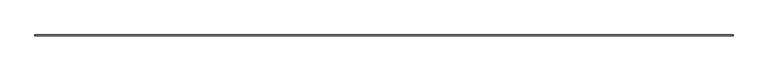
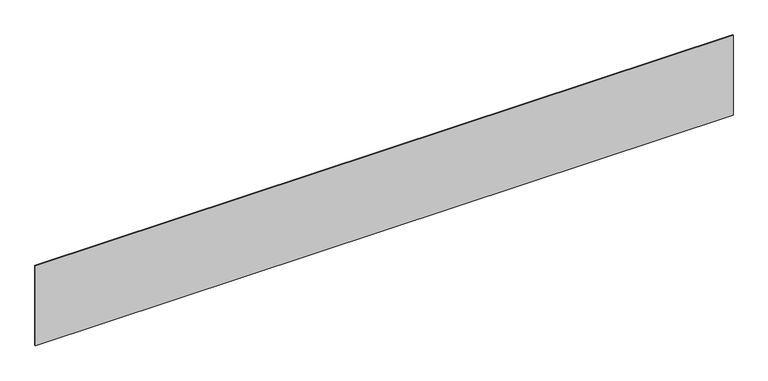
"""IFC4 building model written with IfcOpenShell, lengths in millimetres: proxy geometry, Inner panel:Inner panel:1:Inner panel:1 : Inner panel:Inner panel:300324:300043:Inner panel:1:Inner panel:1 : Inner panel:Inner panel:300324:300043 : Inner panel:Inner panel:1:Inner panel:1 : Inner panel:Inner panel:300324:300043:12 : Inner panel:Inner panel:1:Inner panel:1 : Inner panel:Inner panel:300324:300043:Inner panel:1:Inner panel:1 : Inner panel:Inner panel:300324:300043 : Inner panel:Inner panel:1:Inner panel:1 : Inner panel:Inner panel:300324:300043:300031."""

from ifc_helpers import new_model, si_unit, frame, origin, place, context, project, spatial, polyline, outline, extrude, source, transform, mapped, element, save


def generic_models_44e0b5d8(model_context):
    return source(origin(), model_context, "Body", "SweptSolid", [
        extrude(outline(polyline([(560352.9617239, -579000.6913841), (570446.2867239, -579000.6913841), (570446.2867239, -579013.3913841), (560352.9617239, -579013.3913841), (560352.9617239, -579000.6913841)])), frame((0.0, 0.0, 3721.1), z_axis=(0.0, 0.0, 1.0), x_axis=(1.0, 0.0, 0.0)), (0.0, 0.0, 1.0), 1219.2),
    ])


if __name__ == "__main__":
    model = new_model("IFC4")
    model_context = context("Model", 3, world=origin())
    ifc_project = project(units=[si_unit("LENGTHUNIT", "METRE", prefix="MILLI")], contexts=[model_context])
    site = spatial("IfcSite", under=ifc_project)
    building = spatial("IfcBuilding", under=site)
    placement = place(None, origin())
    generic_models_shape = generic_models_44e0b5d8(model_context)
    element("IfcBuildingElementProxy", 1, Name="Inner panel:Inner panel:1:Inner panel:1 : Inner panel:Inner panel:300324:300043:Inner panel:1:Inner panel:1 : Inner panel:Inner panel:300324:300043 : Inner panel:Inner panel:1:Inner panel:1 : Inner panel:Inner panel:300324:300043:12 : Inner panel:Inner panel:1:Inner panel:1 : Inner panel:Inner panel:300324:300043:Inner panel:1:Inner panel:1 : Inner panel:Inner panel:300324:300043 : Inner panel:Inner panel:1:Inner panel:1 : Inner panel:Inner panel:300324:300043:300031", ObjectType="Inner panel:Inner panel:1:Inner panel:1 : Inner panel:Inner panel:300324:300043:Inner panel:1:Inner panel:1 : Inner panel:Inner panel:300324:300043 : Inner panel:Inner panel:1:Inner panel:1 : Inner panel:Inner panel:300324:300043:12 : Inner panel:Inner panel:1:Inner panel:1 : Inner panel:Inner panel:300324:300043:Inner panel:1:Inner panel:1 : Inner panel:Inner panel:300324:300043 : Inner panel:Inner panel:1:Inner panel:1 : Inner panel:Inner panel:300324:300043:300031", at=placement, inside=building, context=model_context, shape_type="MappedRepresentation", body=[
        mapped(generic_models_shape, transform((0.0, 0.0, 0.0), x_axis=(1.0, 0.0, 0.0), y_axis=(0.0, 1.0, 0.0), z_axis=(0.0, 0.0, 1.0))),
    ])
    save(model, "model.ifc")

# Revit data of these elements
# Type "Inner panel:Inner panel:1:Inner panel:1 : Inner panel:Inner panel:300324:300043:Inner panel:1:Inner panel:1 : Inner panel:Inner panel:300324:300043 : Inner panel:Inner panel:1:Inner panel:1 : Inner panel:Inner panel:300324:300043:12 : Inner panel:Inner panel:1:Inner panel:1 : Inner panel:Inner panel:300324:300043:Inner panel:1:Inner panel:1 : Inner panel:Inner panel:300324:300043 : Inner panel:Inner panel:1:Inner panel:1 : Inner panel:Inner panel:300324:300043:300031"
#   NameOverride = "Inner panel:Inner panel:1:Inner panel:1 : Inner panel:Inner panel:300324:300043:Inner panel:1:Inner panel:1 : Inner panel:Inner panel:300324:300043 : Inner panel:Inner panel:1:Inner panel:1 : Inner panel:Inner panel:300324:300043:300031"
#   ObjectTypeOverride = "Inner panel:1:Inner panel:1 : Inner panel:Inner panel:300324:300043 : Inner panel:Inner panel:1:Inner panel:1 : Inner panel:Inner panel:300324:300043"
#   Reference = "Inner panel"
#   Tag = "300031"
# Element 1 (IfcBuildingElementProxy, "Inner panel:Inner panel:1:Inner panel:1 : Inner panel:Inner panel:300324:300043:Inner panel:1:Inner panel:1 : Inner panel:Inner panel:300324:300043 : Inner panel:Inner panel:1:Inner panel:1 : Inner panel:Inner panel:300324:300043:12 : Inner panel:Inner panel:1:Inner panel:1 : Inner panel:Inner panel:300324:300043:Inner panel:1:Inner panel:1 : Inner panel:Inner panel:300324:300043 : Inner panel:Inner panel:1:Inner panel:1 : Inner panel:Inner panel:300324:300043:300031")
#   Materials on its faces: "1/2\" FIBERGLASS MAT GYPSUM PANELS"
# Materials
#   "1/2\" FIBERGLASS MAT GYPSUM PANELS": class "Generic", colour RGB 171 170 168, transparency 0, Description = "Gypsum Wall Board", Cost = 0
